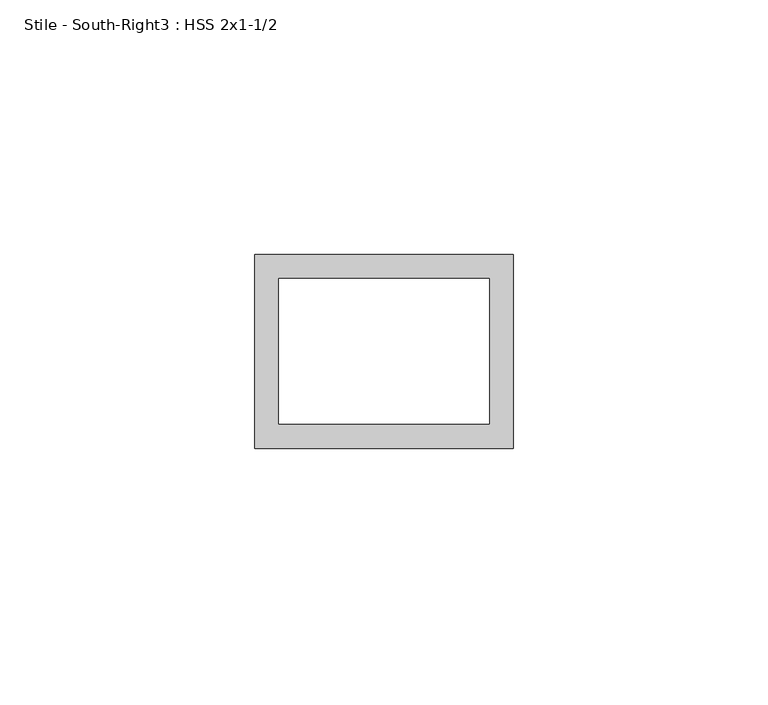
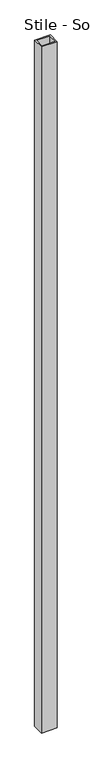
"""IFC4 building model written with IfcOpenShell, lengths in millimetres: proxy geometry, Stile - South-Right3 : HSS 2x1-1/2."""

from ifc_helpers import new_model, si_unit, frame, origin, place, context, project, spatial, polyline, outline, extrude, source, transform, mapped, element, save


def stile_south_right3_hss_2x1_1_2_42ef625e(model_context):
    return source(origin(), model_context, "Body", "SweptSolid", [
        extrude(outline(polyline([(587365.8934739, -536263.6038841), (587416.6934739, -536263.6038841), (587416.6934739, -536301.7038841), (587365.8934739, -536301.7038841), (587365.8934739, -536263.6038841)]), holes=[polyline([(587370.6559739, -536268.3663841), (587370.6559739, -536296.9413841), (587411.9309739, -536296.9413841), (587411.9309739, -536268.3663841), (587370.6559739, -536268.3663841)])]), frame((0.0, 0.0, 50.8), z_axis=(0.0, 0.0, 1.0), x_axis=(1.0, 0.0, 0.0)), (0.0, 0.0, 1.0), 2349.5),
    ])


if __name__ == "__main__":
    model = new_model("IFC4")
    model_context = context("Model", 3, world=origin())
    ifc_project = project(units=[si_unit("LENGTHUNIT", "METRE", prefix="MILLI")], contexts=[model_context])
    site = spatial("IfcSite", under=ifc_project)
    building = spatial("IfcBuilding", under=site)
    placement = place(None, origin())
    stile_south_right3_hss_2x1_1_2_shape = stile_south_right3_hss_2x1_1_2_42ef625e(model_context)
    element("IfcBuildingElementProxy", 1, Name="Stile - South-Right3 : HSS 2x1-1/2", ObjectType="Stile - South-Right3 : HSS 2x1-1/2", at=placement, inside=building, context=model_context, shape_type="MappedRepresentation", body=[
        mapped(stile_south_right3_hss_2x1_1_2_shape, transform((0.0, 0.0, 0.0), x_axis=(1.0, 0.0, 0.0), y_axis=(0.0, 1.0, 0.0), z_axis=(0.0, 0.0, 1.0))),
    ])
    save(model, "model.ifc")

# Revit data of these elements
# Element 1 (IfcBuildingElementProxy, "Stile - South-Right3 : HSS 2x1-1/2")
#   Materials on its faces: "1-1/2\"X2\" GALV. STL HSS TUBING"
# Materials
#   "1-1/2\"X2\" GALV. STL HSS TUBING": class "Generic", colour RGB 211 211 207, transparency 0, Cost = 0
